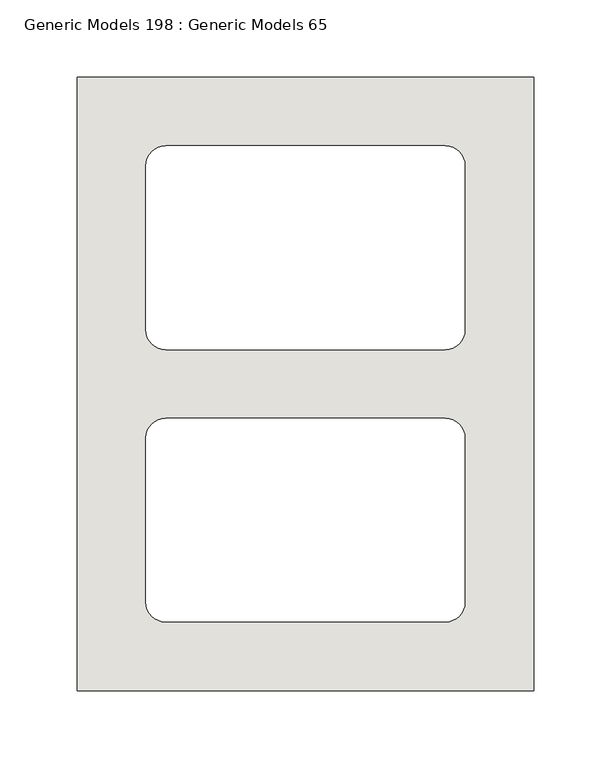
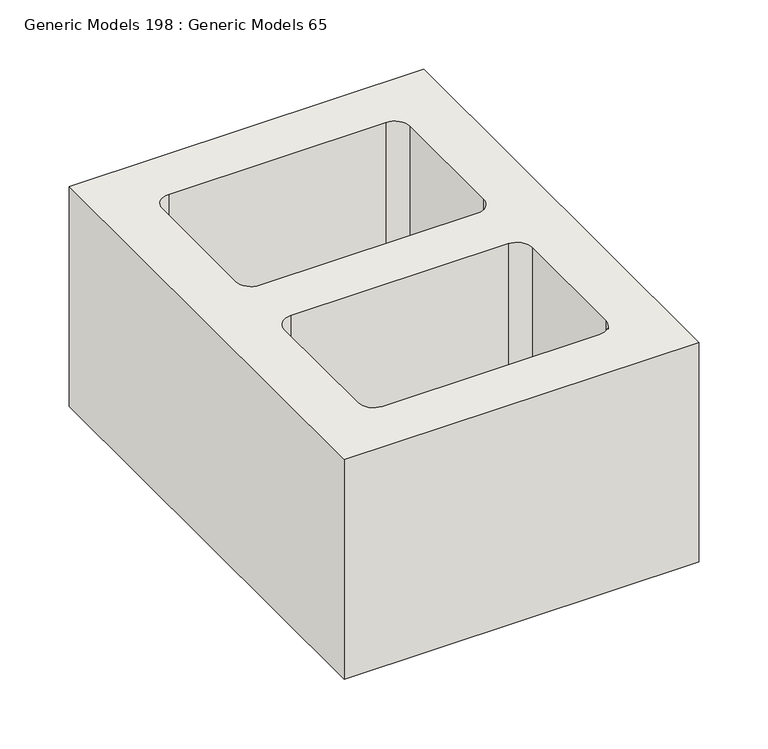
"""IFC4 building model written with IfcOpenShell, lengths in millimetres: wall geometry, Generic Models 198 : Generic Models 65."""

from ifc_helpers import new_model, si_unit, point, frame, frame_2d, origin, place, context, project, spatial, polyline, circle_curve, trimmed, segment, composite_curve, outline, extrude, source, transform, mapped, element, save


def generic_models_198_generic_models_65_1985b1eb(model_context):
    return source(origin(), model_context, "Body", "SweptSolid", [
        extrude(outline(polyline([(748323.2916733, 292.1), (748028.0166733, 292.1), (748028.0166733, 688.975), (748323.2916733, 688.975), (748323.2916733, 292.1)]), holes=[composite_curve([segment(polyline([(748278.8416733, 525.4625), (748278.8416733, 631.825)]), True, "CONTINUOUS"), segment(trimmed(circle_curve(frame_2d((748266.1416733, 631.825)), 12.7), [point((748278.8416733, 631.825))], [point((748266.1416733, 644.525))], True, "CARTESIAN"), True, "CONTINUOUS"), segment(polyline([(748266.1416733, 644.525), (748085.1666733, 644.525)]), True, "CONTINUOUS"), segment(trimmed(circle_curve(frame_2d((748085.1666733, 631.825)), 12.7), [point((748085.1666733, 644.525))], [point((748072.4666733, 631.825))], True, "CARTESIAN"), True, "CONTINUOUS"), segment(polyline([(748072.4666733, 631.825), (748072.4666733, 525.4625)]), True, "CONTINUOUS"), segment(trimmed(circle_curve(frame_2d((748085.1666733, 525.4625)), 12.7), [point((748072.4666733, 525.4625))], [point((748085.1666733, 512.7625))], True, "CARTESIAN"), True, "CONTINUOUS"), segment(polyline([(748085.1666733, 512.7625), (748266.1416733, 512.7625)]), True, "CONTINUOUS"), segment(trimmed(circle_curve(frame_2d((748266.1416733, 525.4625)), 12.7), [point((748266.1416733, 512.7625))], [point((748278.8416733, 525.4625))], True, "CARTESIAN"), True, "CONTINUOUS")], self_intersect=False), composite_curve([segment(polyline([(748072.4666733, 455.6125), (748072.4666733, 349.25)]), True, "CONTINUOUS"), segment(trimmed(circle_curve(frame_2d((748085.1666733, 349.25)), 12.7), [point((748072.4666733, 349.25))], [point((748085.1666733, 336.55))], True, "CARTESIAN"), True, "CONTINUOUS"), segment(polyline([(748085.1666733, 336.55), (748266.1416733, 336.55)]), True, "CONTINUOUS"), segment(trimmed(circle_curve(frame_2d((748266.1416733, 349.25)), 12.7), [point((748266.1416733, 336.55))], [point((748278.8416733, 349.25))], True, "CARTESIAN"), True, "CONTINUOUS"), segment(polyline([(748278.8416733, 349.25), (748278.8416733, 455.6125)]), True, "CONTINUOUS"), segment(trimmed(circle_curve(frame_2d((748266.1416733, 455.6125)), 12.7), [point((748278.8416733, 455.6125))], [point((748266.1416733, 468.3125))], True, "CARTESIAN"), True, "CONTINUOUS"), segment(polyline([(748266.1416733, 468.3125), (748085.1666733, 468.3125)]), True, "CONTINUOUS"), segment(trimmed(circle_curve(frame_2d((748085.1666733, 455.6125)), 12.7), [point((748085.1666733, 468.3125))], [point((748072.4666733, 455.6125))], True, "CARTESIAN"), True, "CONTINUOUS")], self_intersect=False)]), frame((0.0, 0.0, 2195.2893918), z_axis=(0.0, 0.0, 1.0), x_axis=(1.0, 0.0, 0.0)), (0.0, 0.0, 1.0), 193.675),
    ])


if __name__ == "__main__":
    model = new_model("IFC4")
    model_context = context("Model", 3, world=origin())
    ifc_project = project(units=[si_unit("LENGTHUNIT", "METRE", prefix="MILLI")], contexts=[model_context])
    site = spatial("IfcSite", under=ifc_project)
    building = spatial("IfcBuilding", under=site)
    placement = place(None, origin())
    generic_models_198_generic_models_65_shape = generic_models_198_generic_models_65_1985b1eb(model_context)
    element("IfcWall", 1, ObjectType="Generic Models 198 : Generic Models 65", at=placement, inside=building, context=model_context, shape_type="MappedRepresentation", body=[
        mapped(generic_models_198_generic_models_65_shape, transform((0.0, 0.0, 0.0), x_axis=(1.0, 0.0, 0.0), y_axis=(0.0, 1.0, 0.0), z_axis=(0.0, 0.0, 1.0))),
    ])
    save(model, "model.ifc")

# Revit data of these elements
# Element 1 (IfcWall, "Generic Models 198 : Generic Models 65")
#   Materials on its faces: "CONT. KNOCK OUT BOND BEAM"
# Materials
#   "CONT. KNOCK OUT BOND BEAM": class "Masonry", colour RGB 203 203 199, transparency 0, Description = "Concrete masonry units", Cost = 0
